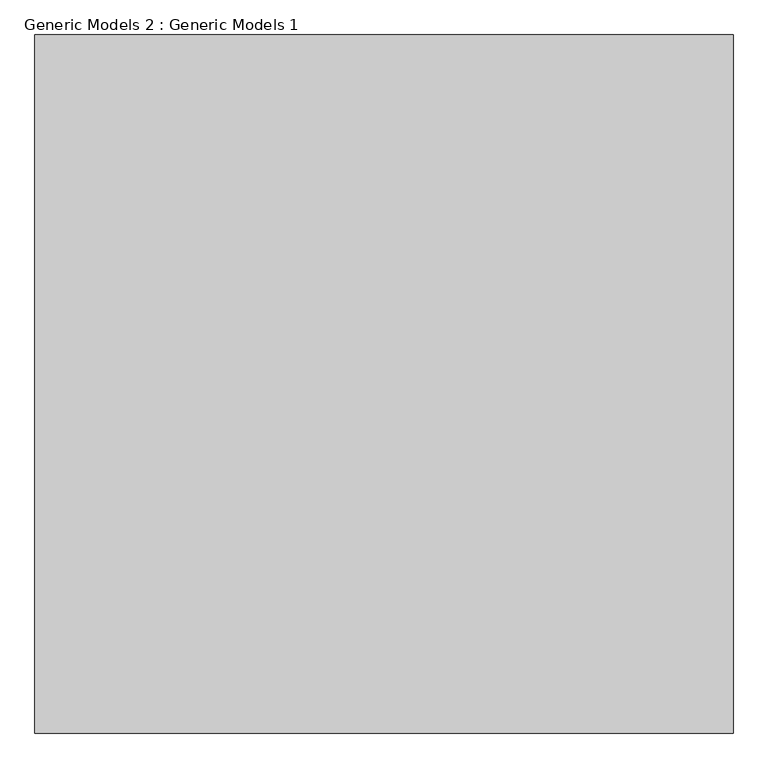
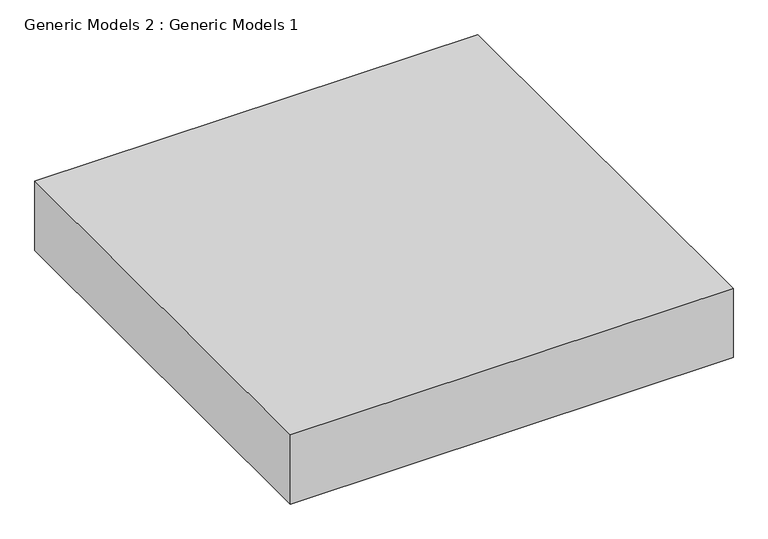
"""IFC4 building model written with IfcOpenShell, lengths in millimetres: proxy geometry, Generic Models 2 : Generic Models 1."""

from ifc_helpers import new_model, si_unit, origin, origin_with_axes, place, context, project, spatial, polyline, outline, extrude, source, transform, mapped, element, save


def generic_models_2_generic_models_1_e905d6e5(model_context):
    return source(origin(), model_context, "Body", "SweptSolid", [
        extrude(outline(polyline([(1524.0, 0.0), (0.0, 0.0), (0.0, 1524.0), (1524.0, 1524.0), (1524.0, 0.0)])), origin_with_axes(), (0.0, 0.0, 1.0), 251.7092939),
    ])


if __name__ == "__main__":
    model = new_model("IFC4")
    model_context = context("Model", 3, world=origin())
    ifc_project = project(units=[si_unit("LENGTHUNIT", "METRE", prefix="MILLI")], contexts=[model_context])
    site = spatial("IfcSite", under=ifc_project)
    building = spatial("IfcBuilding", under=site)
    placement = place(None, origin())
    generic_models_2_generic_models_1_shape = generic_models_2_generic_models_1_e905d6e5(model_context)
    element("IfcBuildingElementProxy", 1, Name="Generic Models 2 : Generic Models 1", ObjectType="Generic Models 2 : Generic Models 1", at=placement, inside=building, context=model_context, shape_type="MappedRepresentation", body=[
        mapped(generic_models_2_generic_models_1_shape, transform((0.0, 0.0, 0.0), x_axis=(1.0, 0.0, 0.0), y_axis=(0.0, 1.0, 0.0), z_axis=(0.0, 0.0, 1.0))),
    ])
    save(model, "model.ifc")
